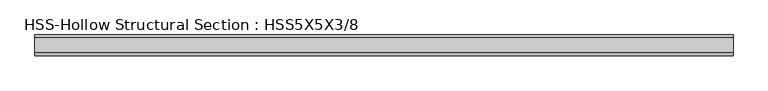
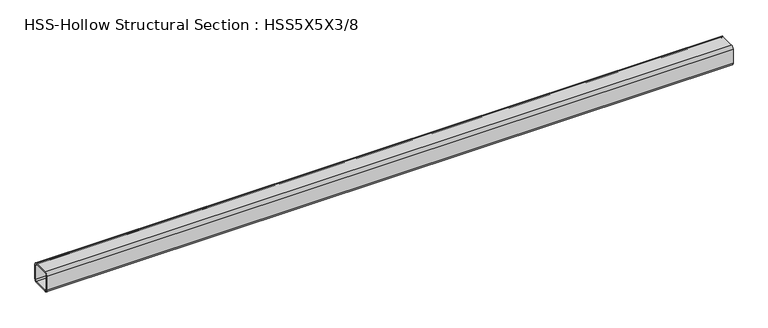
"""IFC4 building model written with IfcOpenShell, lengths in millimetres: beam geometry, HSS-Hollow Structural Section : HSS5X5X3/8."""

from ifc_helpers import new_model, si_unit, point, frame, frame_2d, origin, place, context, project, spatial, polyline, circle_curve, trimmed, segment, composite_curve, outline, extrude, source, transform, mapped, element, save


def hss_hollow_structural_section_hss5x5x3_8_2a917928(model_context):
    return source(origin(), model_context, "Body", "SweptSolid", [
        extrude(outline(composite_curve([segment(trimmed(circle_curve(frame_2d((-45.7708, 45.7708)), 17.7292), [point((-63.5, 45.7708))], [point((-45.7708, 63.5))], False, "CARTESIAN"), True, "CONTINUOUS"), segment(polyline([(-45.7708, 63.5), (45.7708, 63.5)]), True, "CONTINUOUS"), segment(trimmed(circle_curve(frame_2d((45.7708, 45.7708)), 17.7292), [point((45.7708, 63.5))], [point((63.5, 45.7708))], False, "CARTESIAN"), True, "CONTINUOUS"), segment(polyline([(63.5, 45.7708), (63.5, -45.7708)]), True, "CONTINUOUS"), segment(trimmed(circle_curve(frame_2d((45.7708, -45.7708)), 17.7292), [point((63.5, -45.7708))], [point((45.7708, -63.5))], False, "CARTESIAN"), True, "CONTINUOUS"), segment(polyline([(45.7708, -63.5), (-45.7708, -63.5)]), True, "CONTINUOUS"), segment(trimmed(circle_curve(frame_2d((-45.7708, -45.7708)), 17.7292), [point((-45.7708, -63.5))], [point((-63.5, -45.7708))], False, "CARTESIAN"), True, "CONTINUOUS"), segment(polyline([(-63.5, -45.7708), (-63.5, 45.7708)]), True, "CONTINUOUS")], self_intersect=False), holes=[composite_curve([segment(polyline([(45.7708, 54.6354), (-45.7708, 54.6354)]), True, "CONTINUOUS"), segment(trimmed(circle_curve(frame_2d((-45.7708, 45.7708)), 8.8646), [point((-45.7708, 54.6354))], [point((-54.6354, 45.7708))], True, "CARTESIAN"), True, "CONTINUOUS"), segment(polyline([(-54.6354, 45.7708), (-54.6354, -45.7708)]), True, "CONTINUOUS"), segment(trimmed(circle_curve(frame_2d((-45.7708, -45.7708)), 8.8646), [point((-54.6354, -45.7708))], [point((-45.7708, -54.6354))], True, "CARTESIAN"), True, "CONTINUOUS"), segment(polyline([(-45.7708, -54.6354), (45.7708, -54.6354)]), True, "CONTINUOUS"), segment(trimmed(circle_curve(frame_2d((45.7708, -45.7708)), 8.8646), [point((45.7708, -54.6354))], [point((54.6354, -45.7708))], True, "CARTESIAN"), True, "CONTINUOUS"), segment(polyline([(54.6354, -45.7708), (54.6354, 45.7708)]), True, "CONTINUOUS"), segment(trimmed(circle_curve(frame_2d((45.7708, 45.7708)), 8.8646), [point((54.6354, 45.7708))], [point((45.7708, 54.6354))], True, "CARTESIAN"), True, "CONTINUOUS")], self_intersect=False)]), frame((-2120.9, 0.0, 0.0), z_axis=(1.0, 0.0, 0.0), x_axis=(0.0, 1.0, 0.0)), (0.0, 0.0, 1.0), 4241.8),
    ])


if __name__ == "__main__":
    model = new_model("IFC4")
    model_context = context("Model", 3, world=origin())
    ifc_project = project(units=[si_unit("LENGTHUNIT", "METRE", prefix="MILLI")], contexts=[model_context])
    site = spatial("IfcSite", under=ifc_project)
    building = spatial("IfcBuilding", under=site)
    placement = place(None, origin())
    hss_hollow_structural_section_hss5x5x3_8_shape = hss_hollow_structural_section_hss5x5x3_8_2a917928(model_context)
    element("IfcBeam", 1, ObjectType="HSS-Hollow Structural Section : HSS5X5X3/8", at=placement, inside=building, context=model_context, shape_type="MappedRepresentation", body=[
        mapped(hss_hollow_structural_section_hss5x5x3_8_shape, transform((0.0, 0.0, 0.0), x_axis=(1.0, 0.0, 0.0), y_axis=(0.0, 1.0, 0.0), z_axis=(0.0, 0.0, 1.0))),
    ])
    save(model, "model.ifc")

# Revit data of these elements
# Type "HSS-Hollow Structural Section : HSS5X5X3/8"
#   Assembly Code = "B10"
#   Shape = "Square"
#   W = 22.3
#   Ht = 0' - 5"
#   Length [instance default] = 5' - 0"
#   b = 0' - 5"
#   kr = 0' - 0.698"
#   t = 0' - 0.349"
#   A = 0.0429167 SF
#   Structural Material [instance default] = Steel ASTM A500, Grade B, Rectangular and Square
# Element 1 (IfcBeam, "HSS-Hollow Structural Section : HSS5X5X3/8")
#   Materials on its faces: "Steel ASTM A500, Grade B, Rectangular and Square"
# Materials
#   "Steel ASTM A500, Grade B, Rectangular and Square": class "Metal", colour RGB 199 199 199, transparency 0, Description = "Carbon steel", Cost = 0
